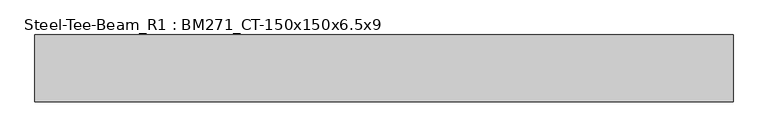
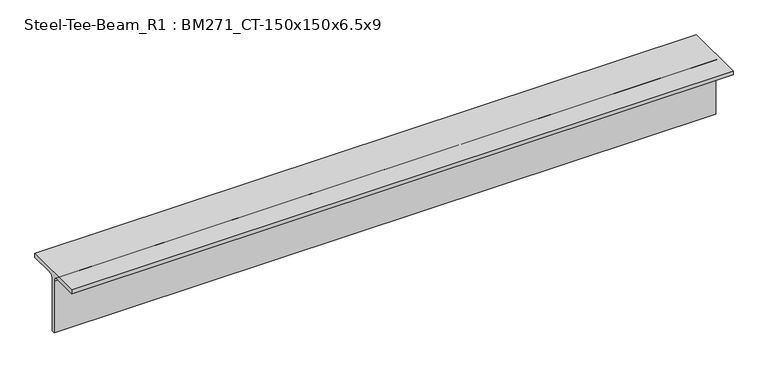
"""IFC4 building model written with IfcOpenShell, lengths in millimetres: member geometry, Steel-Tee-Beam_R1 : BM271_CT-150x150x6.5x9."""

from ifc_helpers import new_model, si_unit, point, frame, frame_2d, origin, place, context, project, spatial, polyline, circle_curve, trimmed, segment, composite_curve, outline, extrude, source, transform, mapped, element, save


def steel_tee_beam_r1_bm271_ct_150x150x6_5x9_5af65525(model_context):
    return source(origin(), model_context, "Body", "SweptSolid", [
        extrude(outline(composite_curve([segment(polyline([(75.0, 75.0), (75.0, 66.0), (16.25, 66.0)]), True, "CONTINUOUS"), segment(trimmed(circle_curve(frame_2d((16.25, 53.0)), 13.0), [point((16.25, 66.0))], [point((3.25, 53.0))], True, "CARTESIAN"), True, "CONTINUOUS"), segment(polyline([(3.25, 53.0), (3.25, -75.0), (-3.25, -75.0), (-3.25, 53.0)]), True, "CONTINUOUS"), segment(trimmed(circle_curve(frame_2d((-16.25, 53.0)), 13.0), [point((-3.25, 53.0))], [point((-16.25, 66.0))], True, "CARTESIAN"), True, "CONTINUOUS"), segment(polyline([(-16.25, 66.0), (-75.0, 66.0), (-75.0, 75.0), (75.0, 75.0)]), True, "CONTINUOUS")], self_intersect=False)), frame((-860.2325267, 0.0, 0.0), z_axis=(1.0, 0.0, 0.0), x_axis=(0.0, 1.0, 0.0)), (0.0, 0.0, 1.0), 1562.0258541),
    ])


if __name__ == "__main__":
    model = new_model("IFC4")
    model_context = context("Model", 3, world=origin())
    ifc_project = project(units=[si_unit("LENGTHUNIT", "METRE", prefix="MILLI")], contexts=[model_context])
    site = spatial("IfcSite", under=ifc_project)
    building = spatial("IfcBuilding", under=site)
    placement = place(None, origin())
    steel_tee_beam_r1_bm271_ct_150x150x6_5x9_shape = steel_tee_beam_r1_bm271_ct_150x150x6_5x9_5af65525(model_context)
    element("IfcMember", 1, ObjectType="Steel-Tee-Beam_R1 : BM271_CT-150x150x6.5x9", at=placement, inside=building, context=model_context, shape_type="MappedRepresentation", body=[
        mapped(steel_tee_beam_r1_bm271_ct_150x150x6_5x9_shape, transform((0.0, 0.0, 0.0), x_axis=(1.0, 0.0, 0.0), y_axis=(0.0, 1.0, 0.0), z_axis=(0.0, 0.0, 1.0))),
    ])
    save(model, "model.ifc")

# Revit data of these elements
# Type "Steel-Tee-Beam_R1 : BM271_CT-150x150x6.5x9"
#   Keynote = "CT-150x150x6.5x9"
#   Surface Area = 0.588841 m²/m
#   Section Area = 23.3904 cm²
#   Mass per Unit Length = 18.3614 kg/m
#   Length [instance default] = 1.5240 m
#   bf = 0.1500 m
#   d = 0.1500 m
#   k = 0.0220 m
#   r = 0.0130 m
#   tf = 0.0090 m
#   tw = 0.0065 m
#   hec_material4 [instance default] = none
#   hec_material3 [instance default] = none
#   hec_material2 [instance default] = none
#   hec_material1 [instance default] = none
#   Structural Material [instance default] = Steel, 45-345
#   Assembly Code = ""
# Element 1 (IfcMember, "Steel-Tee-Beam_R1 : BM271_CT-150x150x6.5x9")
#   Structural Material = none
# Materials
#   "Steel, 45-345": class "Metal", colour RGB 189 187 185, transparency 0, Description = "Steel 345 MPa", Cost = 0
